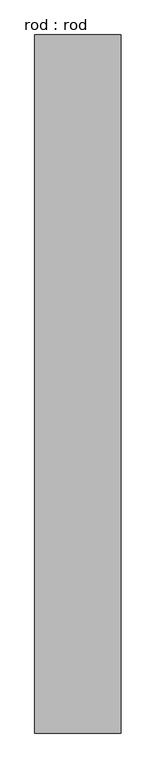
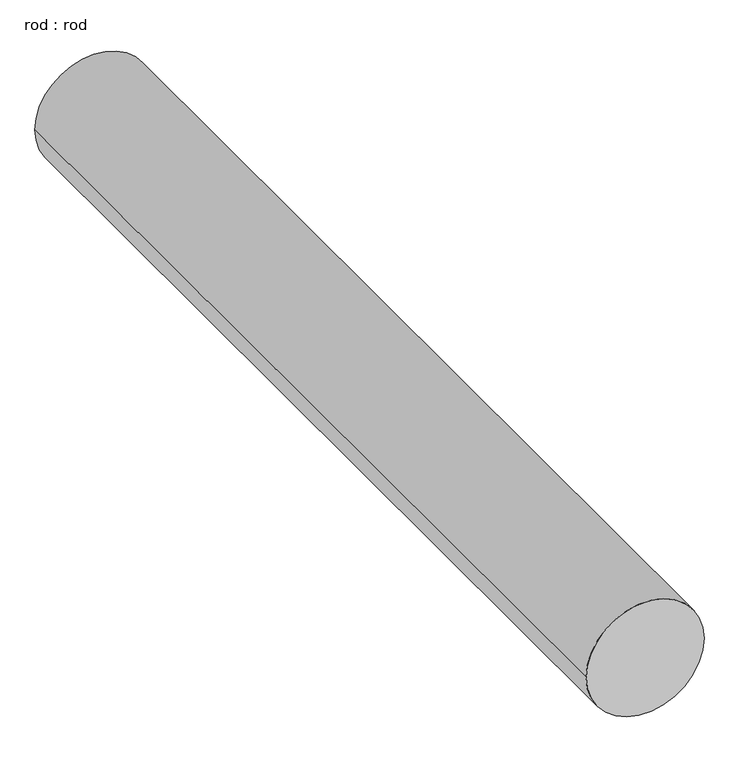
"""IFC4 building model written with IfcOpenShell, lengths in millimetres: proxy geometry, rod : rod."""

from ifc_helpers import new_model, si_unit, point, frame, frame_2d, origin, place, context, project, spatial, circle_curve, trimmed, segment, composite_curve, outline, extrude, source, transform, mapped, element, save


def rod_rod_72d5528f(model_context):
    return source(origin(), model_context, "Body", "SweptSolid", [
        extrude(outline(composite_curve([segment(trimmed(circle_curve(frame_2d((0.0108462, 0.0)), 200.0), [point((0.0108462, 200.0))], [point((0.0108462, -200.0))], False, "CARTESIAN"), True, "CONTINUOUS"), segment(trimmed(circle_curve(frame_2d((0.0108462, 0.0)), 200.0), [point((0.0108462, -200.0))], [point((0.0108462, 200.0))], False, "CARTESIAN"), True, "CONTINUOUS")], self_intersect=False)), frame((0.0, 2472.7286153, 0.0), z_axis=(0.0, 1.0, 0.0), x_axis=(0.0, 0.0, 1.0)), (0.0, 0.0, 1.0), 3240.0),
    ])


if __name__ == "__main__":
    model = new_model("IFC4")
    model_context = context("Model", 3, world=origin())
    ifc_project = project(units=[si_unit("LENGTHUNIT", "METRE", prefix="MILLI")], contexts=[model_context])
    site = spatial("IfcSite", under=ifc_project)
    building = spatial("IfcBuilding", under=site)
    placement = place(None, origin())
    rod_rod_shape = rod_rod_72d5528f(model_context)
    element("IfcBuildingElementProxy", 1, Name="rod : rod", ObjectType="rod : rod", at=placement, inside=building, context=model_context, shape_type="MappedRepresentation", body=[
        mapped(rod_rod_shape, transform((0.0, 0.0, 0.0), x_axis=(1.0, 0.0, 0.0), y_axis=(0.0, 1.0, 0.0), z_axis=(0.0, 0.0, 1.0))),
    ])
    save(model, "model.ifc")

# Revit data of these elements
# Type "rod : rod"
#   Default Elevation = 0
